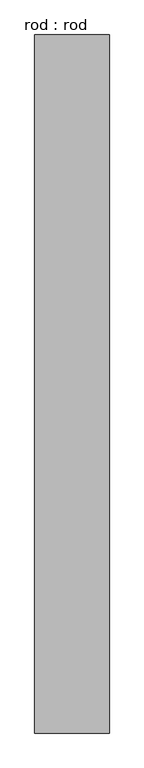
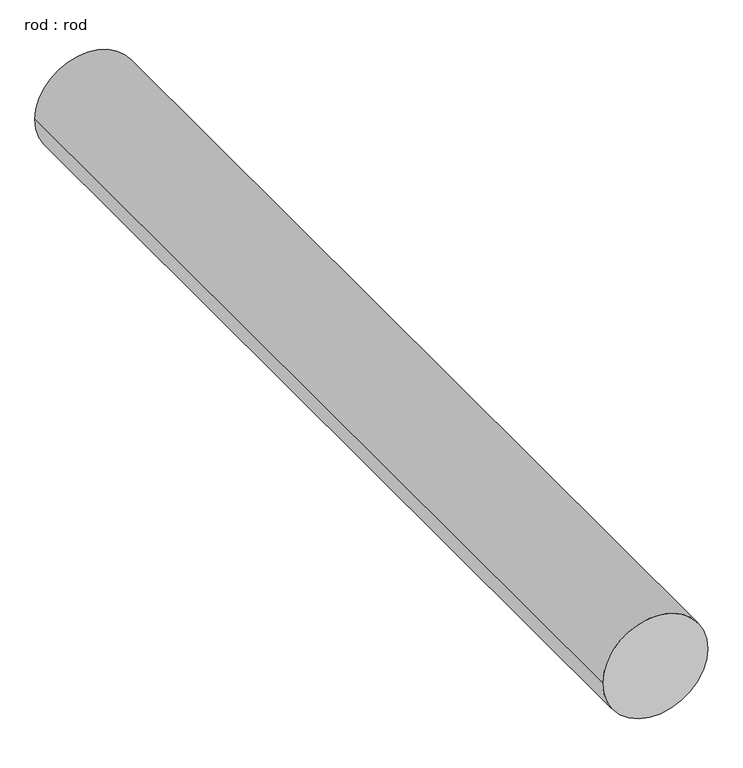
"""IFC4 building model written with IfcOpenShell, lengths in millimetres: proxy geometry, rod : rod."""

from ifc_helpers import new_model, si_unit, point, frame, frame_2d, origin, place, context, project, spatial, circle_curve, trimmed, segment, composite_curve, outline, extrude, source, transform, mapped, element, save


def rod_rod_3274e91e(model_context):
    return source(origin(), model_context, "Body", "SweptSolid", [
        extrude(outline(composite_curve([segment(trimmed(circle_curve(frame_2d((0.0108462, 0.0)), 200.0), [point((0.0108462, 200.0))], [point((0.0108462, -200.0))], False, "CARTESIAN"), True, "CONTINUOUS"), segment(trimmed(circle_curve(frame_2d((0.0108462, 0.0)), 200.0), [point((0.0108462, -200.0))], [point((0.0108462, 200.0))], False, "CARTESIAN"), True, "CONTINUOUS")], self_intersect=False)), frame((0.0, 2221.8581628, 0.0), z_axis=(0.0, 1.0, 0.0), x_axis=(0.0, 0.0, 1.0)), (0.0, 0.0, 1.0), 3741.740905),
    ])


if __name__ == "__main__":
    model = new_model("IFC4")
    model_context = context("Model", 3, world=origin())
    ifc_project = project(units=[si_unit("LENGTHUNIT", "METRE", prefix="MILLI")], contexts=[model_context])
    site = spatial("IfcSite", under=ifc_project)
    building = spatial("IfcBuilding", under=site)
    placement = place(None, origin())
    rod_rod_shape = rod_rod_3274e91e(model_context)
    element("IfcBuildingElementProxy", 1, Name="rod : rod", ObjectType="rod : rod", at=placement, inside=building, context=model_context, shape_type="MappedRepresentation", body=[
        mapped(rod_rod_shape, transform((0.0, 0.0, 0.0), x_axis=(1.0, 0.0, 0.0), y_axis=(0.0, 1.0, 0.0), z_axis=(0.0, 0.0, 1.0))),
    ])
    save(model, "model.ifc")

# Revit data of these elements
# Type "rod : rod"
#   Default Elevation = 0
